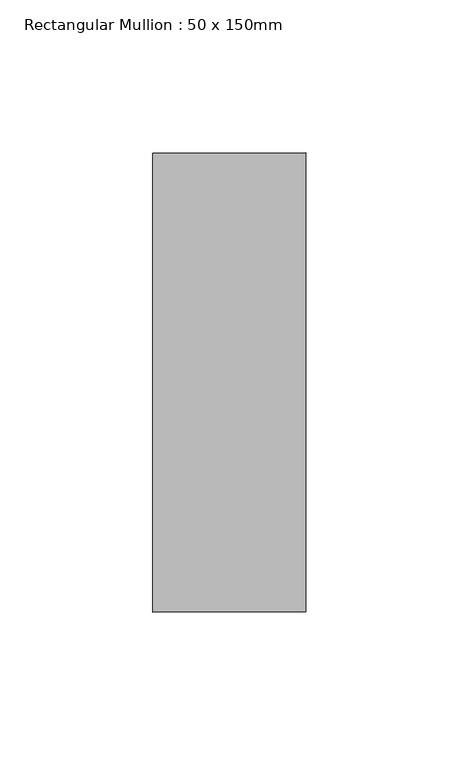
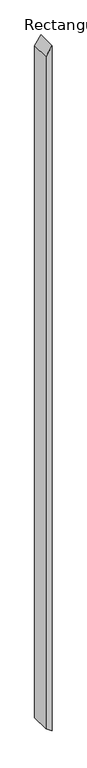
"""IFC4 building model written with IfcOpenShell, lengths in millimetres: member geometry, Rectangular Mullion : 50 x 150mm."""

from ifc_helpers import new_model, si_unit, frame, origin, place, context, project, spatial, polyline, outline, extrude, source, transform, mapped, element, save


def rectangular_mullion_50_x_150mm_2c60866a(model_context):
    return source(origin(), model_context, "Body", "SweptSolid", [
        extrude(outline(polyline([(0.0, 0.0), (-71.6218739, -50.0), (-5613.3621531, -50.0), (-5648.2676905, 0.0), (0.0, 0.0)])), frame((0.0, -75.0, 0.0), z_axis=(0.0, 1.0, 0.0), x_axis=(0.0, 0.0, 1.0)), (0.0, 0.0, 1.0), 150.0),
    ])


if __name__ == "__main__":
    model = new_model("IFC4")
    model_context = context("Model", 3, world=origin())
    ifc_project = project(units=[si_unit("LENGTHUNIT", "METRE", prefix="MILLI")], contexts=[model_context])
    site = spatial("IfcSite", under=ifc_project)
    building = spatial("IfcBuilding", under=site)
    placement = place(None, origin())
    rectangular_mullion_50_x_150mm_shape = rectangular_mullion_50_x_150mm_2c60866a(model_context)
    element("IfcMember", 1, ObjectType="Rectangular Mullion : 50 x 150mm", at=placement, inside=building, context=model_context, shape_type="MappedRepresentation", body=[
        mapped(rectangular_mullion_50_x_150mm_shape, transform((0.0, 0.0, 0.0), x_axis=(1.0, 0.0, 0.0), y_axis=(0.0, 1.0, 0.0), z_axis=(0.0, 0.0, 1.0))),
    ])
    save(model, "model.ifc")

# Revit data of these elements
# Type "Rectangular Mullion : 50 x 150mm"
#   built-in parameter 1007304 = 0.492126 (stored number, unit not read)
#   built-in parameter 1007301 = 0.082021 (stored number, unit not read)
#   built-in parameter 1007300 = 0.082021 (stored number, unit not read)
# Element 1 (IfcMember, "Rectangular Mullion : 50 x 150mm")
#   Materials on its faces: "Metal - Aluminium"
# Materials
#   "Metal - Aluminium": class "Metal", colour RGB 247 247 247, transparency 0
